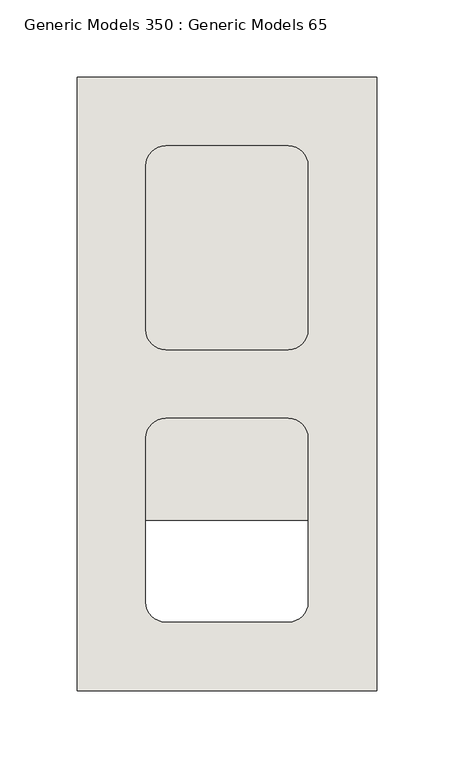
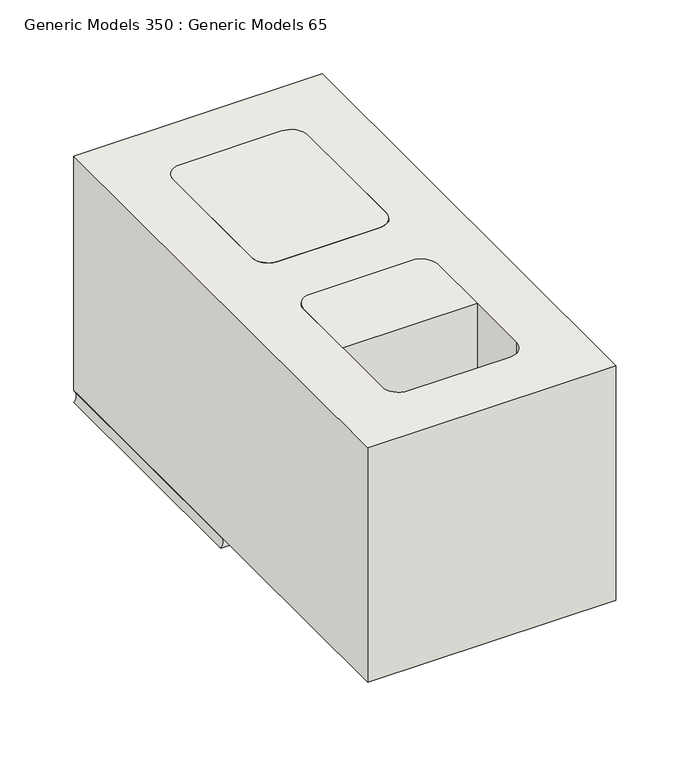
"""IFC4 building model written with IfcOpenShell, lengths in millimetres: wall geometry, Generic Models 350 : Generic Models 65."""

from ifc_helpers import new_model, si_unit, point, frame, frame_2d, origin, place, context, project, spatial, polyline, circle_curve, trimmed, segment, composite_curve, outline, extrude, source, transform, mapped, element, save
from ifc_brep_helpers import plane_surface, revolved_surface, advanced_brep


def generic_models_350_generic_models_65_ba13a9b4(model_context):
    return source(origin(), model_context, "Body", "SolidModel", [
        advanced_brep(
        [(430198.2125, 503.2375, 1431.925), (430004.5375, 503.2375, 1431.925), (430004.5375, 503.2375, 1422.4), (430198.2125, 503.2375, 1422.4), (430198.2125, 701.675, 1431.925), (430198.2125, 701.675, 1422.4), (430004.5375, 701.675, 1422.4), (430004.5375, 701.675, 1431.925), (430153.7625, 538.1625, 1431.925), (430141.0625, 525.4625, 1431.925), (430061.6875, 525.4625, 1431.925), (430048.9875, 538.1625, 1431.925), (430048.9875, 644.525, 1431.925), (430061.6875, 657.225, 1431.925), (430141.0625, 657.225, 1431.925), (430153.7625, 644.525, 1431.925), (430141.0625, 525.4625, 1422.4), (430153.7625, 538.1625, 1422.4), (430061.6875, 525.4625, 1422.4), (430048.9875, 538.1625, 1422.4), (430048.9875, 644.525, 1422.4), (430061.6875, 657.225, 1422.4), (430141.0625, 657.225, 1422.4), (430153.7625, 644.525, 1422.4)],
        [
            (0, 1),
            (1, 2, circle_curve(frame((429999.6545028, 503.2375, 1427.1625), z_axis=(0.0, 1.0, 0.0), x_axis=(1.0, 0.0, 0.0)), 6.8209287)),
            (2, 3),
            (3, 0, circle_curve(frame((430203.0954972, 503.2375, 1427.1625), z_axis=(0.0, 1.0, 0.0), x_axis=(-1.0, 0.0, 0.0)), 6.8209287)),
            (4, 5, circle_curve(frame((430203.0954972, 701.675, 1427.1625), z_axis=(0.0, -1.0, 0.0), x_axis=(-1.0, 0.0, 0.0)), 6.8209287)),
            (5, 6),
            (6, 7, circle_curve(frame((429999.6545028, 701.675, 1427.1625), z_axis=(0.0, -1.0, 0.0), x_axis=(1.0, 0.0, 0.0)), 6.8209287)),
            (7, 4),
            (0, 4),
            (7, 1),
            (8, 9, circle_curve(frame((430141.0625, 538.1625, 1431.925), z_axis=(0.0, 0.0, -1.0), x_axis=(-1.0, 0.0, 0.0)), 12.7)),
            (9, 10),
            (10, 11, circle_curve(frame((430061.6875, 538.1625, 1431.925), z_axis=(0.0, 0.0, -1.0), x_axis=(-1.0, 0.0, 0.0)), 12.7)),
            (11, 12),
            (12, 13, circle_curve(frame((430061.6875, 644.525, 1431.925), z_axis=(0.0, 0.0, -1.0), x_axis=(-1.0, 0.0, 0.0)), 12.7)),
            (13, 14),
            (14, 15, circle_curve(frame((430141.0625, 644.525, 1431.925), z_axis=(0.0, 0.0, -1.0), x_axis=(-1.0, 0.0, 0.0)), 12.7)),
            (15, 8),
            (16, 9),
            (8, 17),
            (17, 16, circle_curve(frame((430141.0625, 538.1625, 1422.4), z_axis=(0.0, 0.0, -1.0), x_axis=(-1.0, 0.0, 0.0)), 12.7)),
            (16, 18),
            (18, 10),
            (18, 19, circle_curve(frame((430061.6875, 538.1625, 1422.4), z_axis=(0.0, 0.0, -1.0), x_axis=(-1.0, 0.0, 0.0)), 12.7)),
            (19, 11),
            (19, 20),
            (20, 12),
            (20, 21, circle_curve(frame((430061.6875, 644.525, 1422.4), z_axis=(0.0, 0.0, -1.0), x_axis=(-1.0, 0.0, 0.0)), 12.7)),
            (21, 13),
            (21, 22),
            (22, 14),
            (22, 23, circle_curve(frame((430141.0625, 644.525, 1422.4), z_axis=(0.0, 0.0, -1.0), x_axis=(-1.0, 0.0, 0.0)), 12.7)),
            (23, 15),
            (23, 17),
            (6, 2),
            (5, 3),
        ],
        [
            plane_surface(frame((430101.375, 503.2375, 1432.321875), z_axis=(0.0, -1.0, 0.0), x_axis=(0.0, 0.0, 1.0))),
            plane_surface(frame((430101.375, 701.675, 1432.321875), z_axis=(0.0, 1.0, 0.0), x_axis=(0.0, 0.0, 1.0))),
            plane_surface(frame((430198.2125, 503.2375, 1431.925), z_axis=(0.0, 0.0, 1.0), x_axis=(0.0, 1.0, 0.0))),
            revolved_surface(polyline([(430128.3625, 538.1625, 1431.925), (430128.3625, 538.1625, 1422.4)]), (430141.0625, 538.1625, 1616.075), (0.0, 0.0, 1.0)),
            plane_surface(frame((430061.6875, 525.4625, 1616.075), z_axis=(0.0, 1.0, 0.0), x_axis=(0.0, 0.0, -1.0))),
            revolved_surface(polyline([(430048.9875, 538.1625, 1431.925), (430048.9875, 538.1625, 1422.4)]), (430061.6875, 538.1625, 1616.075), (0.0, 0.0, 1.0)),
            plane_surface(frame((430048.9875, 644.525, 1616.075), z_axis=(1.0, 0.0, 0.0), x_axis=(0.0, 0.0, -1.0))),
            revolved_surface(polyline([(430048.9875, 644.525, 1431.925), (430048.9875, 644.525, 1422.4)]), (430061.6875, 644.525, 1616.075), (0.0, 0.0, 1.0)),
            plane_surface(frame((430141.0625, 657.225, 1616.075), z_axis=(0.0, -1.0, 0.0), x_axis=(0.0, 0.0, -1.0))),
            revolved_surface(polyline([(430128.3625, 644.525, 1431.925), (430128.3625, 644.525, 1422.4)]), (430141.0625, 644.525, 1616.075), (0.0, 0.0, 1.0)),
            plane_surface(frame((430153.7625, 538.1625, 1616.075), z_axis=(-1.0, 0.0, 0.0), x_axis=(0.0, 0.0, -1.0))),
            revolved_surface(polyline([(430006.4754315, 701.675, 1427.1625), (430006.4754315, 503.2375, 1427.1625)]), (429999.6545028, 503.2375, 1427.1625), (0.0, 1.0, 0.0)),
            plane_surface(frame((430004.5375, 503.2375, 1422.4), z_axis=(0.0, 0.0, -1.0), x_axis=(0.0, 1.0, 0.0))),
            revolved_surface(polyline([(430196.2745685, 701.675, 1427.1625), (430196.2745685, 503.2375, 1427.1625)]), (430203.0954972, 503.2375, 1427.1625), (0.0, 1.0, 0.0)),
        ],
        [
            (0, [[1, 2, 3, 4]]),
            (1, [[5, 6, 7, 8]]),
            (2, [[-1, 9, -8, 10], [11, 12, 13, 14, 15, 16, 17, 18]]),
            (3, [[19, -11, 20, 21]]),
            (4, [[-19, 22, 23, -12]]),
            (5, [[-23, 24, 25, -13]]),
            (6, [[-25, 26, 27, -14]]),
            (7, [[-27, 28, 29, -15]]),
            (8, [[-29, 30, 31, -16]]),
            (9, [[-31, 32, 33, -17]]),
            (10, [[-33, 34, -20, -18]]),
            (11, [[-2, -10, -7, 35]]),
            (12, [[-3, -35, -6, 36], [-21, -34, -32, -30, -28, -26, -24, -22]]),
            (13, [[-4, -36, -5, -9]]),
        ],
    ),
        extrude(outline(composite_curve([segment(trimmed(circle_curve(frame_2d((430141.0625, 538.1625)), 12.7), [point((430153.7625, 538.1625))], [point((430141.0625, 525.4625))], False, "CARTESIAN"), True, "CONTINUOUS"), segment(polyline([(430141.0625, 525.4625), (430061.6875, 525.4625)]), True, "CONTINUOUS"), segment(trimmed(circle_curve(frame_2d((430061.6875, 538.1625)), 12.7), [point((430061.6875, 525.4625))], [point((430048.9875, 538.1625))], False, "CARTESIAN"), True, "CONTINUOUS"), segment(polyline([(430048.9875, 538.1625), (430048.9875, 644.525)]), True, "CONTINUOUS"), segment(trimmed(circle_curve(frame_2d((430061.6875, 644.525)), 12.7), [point((430048.9875, 644.525))], [point((430061.6875, 657.225))], False, "CARTESIAN"), True, "CONTINUOUS"), segment(polyline([(430061.6875, 657.225), (430141.0625, 657.225)]), True, "CONTINUOUS"), segment(trimmed(circle_curve(frame_2d((430141.0625, 644.525)), 12.7), [point((430141.0625, 657.225))], [point((430153.7625, 644.525))], False, "CARTESIAN"), True, "CONTINUOUS"), segment(polyline([(430153.7625, 644.525), (430153.7625, 538.1625)]), True, "CONTINUOUS")], self_intersect=False)), frame((0.0, 0.0, 1422.4), z_axis=(0.0, 0.0, 1.0), x_axis=(1.0, 0.0, 0.0)), (0.0, 0.0, 1.0), 203.2),
        extrude(outline(composite_curve([segment(trimmed(circle_curve(frame_2d((430061.6875, 468.3125)), 12.7), [point((430048.9875, 468.3125))], [point((430061.6875, 481.0125))], False, "CARTESIAN"), True, "CONTINUOUS"), segment(polyline([(430061.6875, 481.0125), (430141.0625, 481.0125)]), True, "CONTINUOUS"), segment(trimmed(circle_curve(frame_2d((430141.0625, 468.3125)), 12.7), [point((430141.0625, 481.0125))], [point((430153.7625, 468.3125))], False, "CARTESIAN"), True, "CONTINUOUS"), segment(polyline([(430153.7625, 468.3125), (430153.7625, 415.13125), (430048.9875, 415.13125), (430048.9875, 468.3125)]), True, "CONTINUOUS")], self_intersect=False)), frame((0.0, 0.0, 1422.4), z_axis=(0.0, 0.0, 1.0), x_axis=(1.0, 0.0, 0.0)), (0.0, 0.0, 1.0), 203.2),
        extrude(outline(polyline([(430198.2125, 304.8), (430004.5375, 304.8), (430004.5375, 701.675), (430198.2125, 701.675), (430198.2125, 304.8)]), holes=[composite_curve([segment(polyline([(430153.7625, 538.1625), (430153.7625, 644.525)]), True, "CONTINUOUS"), segment(trimmed(circle_curve(frame_2d((430141.0625, 644.525)), 12.7), [point((430153.7625, 644.525))], [point((430141.0625, 657.225))], True, "CARTESIAN"), True, "CONTINUOUS"), segment(polyline([(430141.0625, 657.225), (430061.6875, 657.225)]), True, "CONTINUOUS"), segment(trimmed(circle_curve(frame_2d((430061.6875, 644.525)), 12.7), [point((430061.6875, 657.225))], [point((430048.9875, 644.525))], True, "CARTESIAN"), True, "CONTINUOUS"), segment(polyline([(430048.9875, 644.525), (430048.9875, 538.1625)]), True, "CONTINUOUS"), segment(trimmed(circle_curve(frame_2d((430061.6875, 538.1625)), 12.7), [point((430048.9875, 538.1625))], [point((430061.6875, 525.4625))], True, "CARTESIAN"), True, "CONTINUOUS"), segment(polyline([(430061.6875, 525.4625), (430141.0625, 525.4625)]), True, "CONTINUOUS"), segment(trimmed(circle_curve(frame_2d((430141.0625, 538.1625)), 12.7), [point((430141.0625, 525.4625))], [point((430153.7625, 538.1625))], True, "CARTESIAN"), True, "CONTINUOUS")], self_intersect=False), composite_curve([segment(polyline([(430048.9875, 468.3125), (430048.9875, 361.95)]), True, "CONTINUOUS"), segment(trimmed(circle_curve(frame_2d((430061.6875, 361.95)), 12.7), [point((430048.9875, 361.95))], [point((430061.6875, 349.25))], True, "CARTESIAN"), True, "CONTINUOUS"), segment(polyline([(430061.6875, 349.25), (430141.0625, 349.25)]), True, "CONTINUOUS"), segment(trimmed(circle_curve(frame_2d((430141.0625, 361.95)), 12.7), [point((430141.0625, 349.25))], [point((430153.7625, 361.95))], True, "CARTESIAN"), True, "CONTINUOUS"), segment(polyline([(430153.7625, 361.95), (430153.7625, 468.3125)]), True, "CONTINUOUS"), segment(trimmed(circle_curve(frame_2d((430141.0625, 468.3125)), 12.7), [point((430153.7625, 468.3125))], [point((430141.0625, 481.0125))], True, "CARTESIAN"), True, "CONTINUOUS"), segment(polyline([(430141.0625, 481.0125), (430061.6875, 481.0125)]), True, "CONTINUOUS"), segment(trimmed(circle_curve(frame_2d((430061.6875, 468.3125)), 12.7), [point((430061.6875, 481.0125))], [point((430048.9875, 468.3125))], True, "CARTESIAN"), True, "CONTINUOUS")], self_intersect=False)]), frame((0.0, 0.0, 1431.925), z_axis=(0.0, 0.0, 1.0), x_axis=(1.0, 0.0, 0.0)), (0.0, 0.0, 1.0), 193.675),
    ])


if __name__ == "__main__":
    model = new_model("IFC4")
    model_context = context("Model", 3, world=origin())
    ifc_project = project(units=[si_unit("LENGTHUNIT", "METRE", prefix="MILLI")], contexts=[model_context])
    site = spatial("IfcSite", under=ifc_project)
    building = spatial("IfcBuilding", under=site)
    placement = place(None, origin())
    generic_models_350_generic_models_65_shape = generic_models_350_generic_models_65_ba13a9b4(model_context)
    element("IfcWall", 1, ObjectType="Generic Models 350 : Generic Models 65", at=placement, inside=building, context=model_context, shape_type="MappedRepresentation", body=[
        mapped(generic_models_350_generic_models_65_shape, transform((0.0, 0.0, 0.0), x_axis=(1.0, 0.0, 0.0), y_axis=(0.0, 1.0, 0.0), z_axis=(0.0, 0.0, 1.0))),
    ])
    save(model, "model.ifc")

# Revit data of these elements
# Element 1 (IfcWall, "Generic Models 350 : Generic Models 65")
#   Materials on its faces: "CMU (SEE 'WALL TAG' FOR SIZE)", "FILL CORE IF APPLICABLE - SEE STRUCTURAL DWGS FOR DETAILS", "MORTAR JOINT"
# Materials
#   "CMU (SEE 'WALL TAG' FOR SIZE)": class "Masonry", colour RGB 203 203 199, transparency 0, Description = "Concrete masonry units", Cost = 0
#   "FILL CORE IF APPLICABLE - SEE STRUCTURAL DWGS FOR DETAILS": class "Generic", colour RGB 170 170 170, transparency 0, Cost = 0
#   "MORTAR JOINT": class "Generic", colour RGB 120 120 120, transparency 0, Cost = 0
